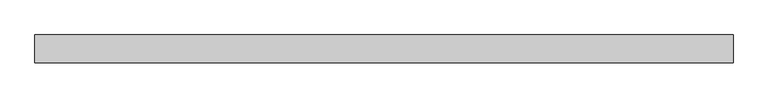
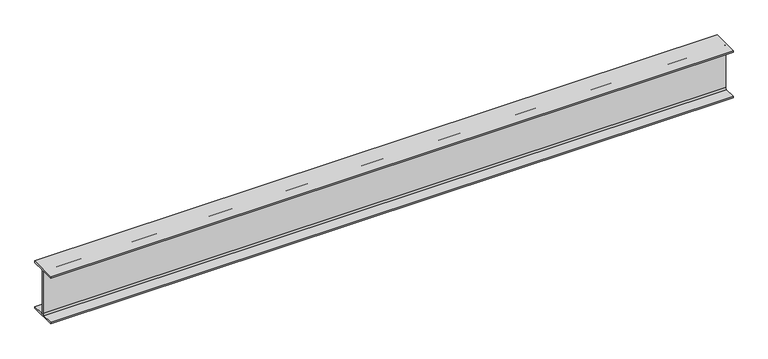
"""IFC4 building model written with IfcOpenShell, lengths in millimetres: beam geometry, Old_Steel Beam_H-KSD3502 : H_SB_ASB_H-250×125x6x9."""

import ifcopenshell
import ifcopenshell.guid

model = None  # the IFC model being written
_history = None  # IfcOwnerHistory: only IFC2X3 demands one
_inside = {}  # id of a spatial element -> (the spatial element, [elements in it])
_under = {}  # id of a project, library or spatial element -> (it, [spatial elements below it])
_declared = {}  # id of a project -> (the project, [libraries it declares])
_typed = {}  # id of a type object -> (the type object, [elements of that type])
_made_of = {}  # id of a material, layer set ... -> (it, [elements and type objects made of it])


def new_model(schema):
    """Start an empty IFC model of exactly this schema.

    Asked for "IFC4X3", IfcOpenShell would pick the latest addendum, in which some entities
    have other attributes; the version numbers below select the first issue.
    IFC2X3 requires an IfcOwnerHistory on every rooted entity: one is made here for all.
    """
    global model, _history
    if schema == "IFC4X3":
        model = ifcopenshell.file(schema_version=(4, 3, 0, 0))
    else:
        model = ifcopenshell.file(schema=schema)
    _inside.clear()
    _under.clear()
    _declared.clear()
    _typed.clear()
    _made_of.clear()
    _history = None
    if model.schema == "IFC2X3":
        org = make("IfcOrganization", Name="unknown")
        user = make(
            "IfcPersonAndOrganization",
            ThePerson=make("IfcPerson", FamilyName="unknown"),
            TheOrganization=org,
        )
        app = make(
            "IfcApplication",
            ApplicationDeveloper=org,
            Version="unknown",
            ApplicationFullName="unknown",
            ApplicationIdentifier="unknown",
        )
        _history = make(
            "IfcOwnerHistory",
            OwningUser=user,
            OwningApplication=app,
            ChangeAction="ADDED",
            CreationDate=0,
        )
    return model


def make(cls, **values):
    """One entity of the class cls with the attributes given. An attribute that is None is left unset."""
    return model.create_entity(
        cls, **{name: value for name, value in values.items() if value is not None}
    )


def rooted(cls, **values):
    """An entity with a GlobalId (a new one), such as an element, a storey or a relation."""
    return make(cls, GlobalId=ifcopenshell.guid.new(), OwnerHistory=_history, **values)


def si_unit(unit_type, name, prefix=None):
    """IfcSIUnit, for example si_unit("LENGTHUNIT", "METRE", prefix="MILLI")."""
    return make("IfcSIUnit", UnitType=unit_type, Prefix=prefix, Name=name)


def assignment(units):
    """IfcUnitAssignment: the units of a project."""
    return None if units is None else make("IfcUnitAssignment", Units=units)


def point(xyz):
    """IfcCartesianPoint."""
    return None if xyz is None else make("IfcCartesianPoint", Coordinates=xyz)


def direction(xyz):
    """IfcDirection."""
    return None if xyz is None else make("IfcDirection", DirectionRatios=xyz)


def frame(location, z_axis=None, x_axis=None):
    """IfcAxis2Placement3D, a coordinate frame: its origin and axes. An axis left out is left unset."""
    return make(
        "IfcAxis2Placement3D",
        Location=point(location),
        Axis=direction(z_axis),
        RefDirection=direction(x_axis),
    )


def frame_2d(location, x_axis=None):
    """IfcAxis2Placement2D, a coordinate frame in the plane: its origin and x axis."""
    return make(
        "IfcAxis2Placement2D", Location=point(location), RefDirection=direction(x_axis)
    )


def origin():
    """The frame at (0, 0, 0) with its axes left unset."""
    return frame((0.0, 0.0, 0.0))


def place(relative_to, where):
    """IfcLocalPlacement: puts the frame where relative to a parent placement (None: the world)."""
    return make(
        "IfcLocalPlacement", PlacementRelTo=relative_to, RelativePlacement=where
    )


def context(
    kind, dimensions, precision=None, world=None, true_north=None, identifier=None
):
    """IfcGeometricRepresentationContext, for example the 3D "Model" context."""
    return make(
        "IfcGeometricRepresentationContext",
        ContextIdentifier=identifier,
        ContextType=kind,
        CoordinateSpaceDimension=dimensions,
        Precision=precision,
        WorldCoordinateSystem=world,
        TrueNorth=true_north,
    )


def project(units=None, contexts=None):
    """IfcProject with its units and contexts."""
    return rooted(
        "IfcProject",
        Name="project",
        RepresentationContexts=contexts,
        UnitsInContext=assignment(units),
    )


def spatial(cls, under=None, at=None, **own):
    """A site, building, storey or space (cls), placed at a placement, below another one or the project."""
    s = rooted(cls, ObjectPlacement=at, **own)
    if under is not None:
        _under.setdefault(under.id(), (under, []))[1].append(s)
    return s


def polyline(points):
    """IfcPolyline through the points."""
    return make("IfcPolyline", Points=[point(p) for p in points])


def circle_curve(where, radius):
    """IfcCircle in the frame where."""
    return make("IfcCircle", Position=where, Radius=radius)


def trimmed(basis, trim1, trim2, sense, master):
    """IfcTrimmedCurve: the piece of a basis curve between two trims."""
    return make(
        "IfcTrimmedCurve",
        BasisCurve=basis,
        Trim1=trim1,
        Trim2=trim2,
        SenseAgreement=sense,
        MasterRepresentation=master,
    )


def segment(curve, same_sense, transition):
    """IfcCompositeCurveSegment."""
    return make(
        "IfcCompositeCurveSegment",
        Transition=transition,
        SameSense=same_sense,
        ParentCurve=curve,
    )


def composite_curve(segments, self_intersect=None):
    """IfcCompositeCurve: segments joined end to end."""
    return make("IfcCompositeCurve", Segments=segments, SelfIntersect=self_intersect)


def outline(outer, holes=None, kind="AREA"):
    """IfcArbitraryClosedProfileDef: a profile drawn as a closed curve; with holes, ...WithVoids."""
    if holes is None:
        return make("IfcArbitraryClosedProfileDef", ProfileType=kind, OuterCurve=outer)
    return make(
        "IfcArbitraryProfileDefWithVoids",
        ProfileType=kind,
        OuterCurve=outer,
        InnerCurves=holes,
    )


def extrude(swept, where, along, depth):
    """IfcExtrudedAreaSolid: the profile swept, set in the frame where, extruded along a direction by depth."""
    return make(
        "IfcExtrudedAreaSolid",
        SweptArea=swept,
        Position=where,
        ExtrudedDirection=direction(along),
        Depth=depth,
    )


def shape(context_of_items, identifier, shape_type, items):
    """IfcShapeRepresentation: the items that make up one representation, for example the "Body"."""
    return make(
        "IfcShapeRepresentation",
        ContextOfItems=context_of_items,
        RepresentationIdentifier=identifier,
        RepresentationType=shape_type,
        Items=items,
    )


def source(mapping_origin, context_of_items, identifier, shape_type, items):
    """IfcRepresentationMap: a shape defined once, which mapped items show again and again."""
    return make(
        "IfcRepresentationMap",
        MappingOrigin=mapping_origin,
        MappedRepresentation=shape(context_of_items, identifier, shape_type, items),
    )


def transform(
    local_origin,
    x_axis=None,
    y_axis=None,
    z_axis=None,
    scale=None,
    scale2=None,
    scale3=None,
    uniform=True,
):
    """IfcCartesianTransformationOperator3D, or its non-uniform kind. x_axis, y_axis, z_axis: its Axis1, 2, 3."""
    if uniform:
        return make(
            "IfcCartesianTransformationOperator3D",
            Axis1=direction(x_axis),
            Axis2=direction(y_axis),
            LocalOrigin=point(local_origin),
            Scale=scale,
            Axis3=direction(z_axis),
        )
    return make(
        "IfcCartesianTransformationOperator3DnonUniform",
        Axis1=direction(x_axis),
        Axis2=direction(y_axis),
        LocalOrigin=point(local_origin),
        Scale=scale,
        Axis3=direction(z_axis),
        Scale2=scale2,
        Scale3=scale3,
    )


def mapped(mapping_source, mapping_target):
    """IfcMappedItem: shows the shape of a source again, moved by a transform."""
    return make(
        "IfcMappedItem", MappingSource=mapping_source, MappingTarget=mapping_target
    )


def made_of(thing, what):
    """Note that an element or type object is made of a material, layer set ...; save() writes the relation."""
    if what is not None:
        _made_of.setdefault(what.id(), (what, []))[1].append(thing)
    return thing


def element(
    cls,
    number,
    at=None,
    inside=None,
    cuts=None,
    type_object=None,
    material=None,
    context=None,
    identifier="Body",
    shape_type=None,
    held_by="IfcProductDefinitionShape",
    body=None,
    shapes=None,
    **own,
):
    """One element of the class cls, such as IfcWall. Its Tag is "e" and its number.

    at: its placement. inside: the storey or other place that contains it. cuts: it is an
    opening in that element (IfcRelVoidsElement). A single representation is given by context,
    identifier, shape_type and body (its items); several are given by shapes. held_by: the class
    of the entity that holds the representations. save() writes the other relations.
    """
    e = rooted(cls, Tag="e%d" % number, ObjectPlacement=at, **own)
    if body is not None:
        shapes = [shape(context, identifier, shape_type, body)]
    if shapes is not None:
        e.Representation = make(held_by, Representations=shapes)
    if inside is not None:
        _inside.setdefault(inside.id(), (inside, []))[1].append(e)
    if cuts is not None:
        rooted(
            "IfcRelVoidsElement", RelatingBuildingElement=cuts, RelatedOpeningElement=e
        )
    if type_object is not None:
        _typed.setdefault(type_object.id(), (type_object, []))[1].append(e)
    return made_of(e, material)


def aggregate(whole, parts):
    """IfcRelAggregates: a whole, such as a stair, and the parts it consists of."""
    return rooted("IfcRelAggregates", RelatingObject=whole, RelatedObjects=parts)


def save(model, path):
    """Write the relations noted so far, then the file.

    IfcRelAggregates (storeys below a building ...), IfcRelContainedInSpatialStructure (elements
    in a storey), IfcRelDefinesByType, IfcRelAssociatesMaterial and IfcRelDeclares: one each for
    every whole, place, type object, material and project.
    """
    for whole, parts in _under.values():
        aggregate(whole, parts)
    for where, things in _inside.values():
        rooted(
            "IfcRelContainedInSpatialStructure",
            RelatedElements=things,
            RelatingStructure=where,
        )
    for kind, things in _typed.values():
        rooted("IfcRelDefinesByType", RelatedObjects=things, RelatingType=kind)
    for what, things in _made_of.values():
        rooted("IfcRelAssociatesMaterial", RelatedObjects=things, RelatingMaterial=what)
    for by, libraries in _declared.values():
        rooted("IfcRelDeclares", RelatingContext=by, RelatedDefinitions=libraries)
    model.write(path)


def beam_10e9c193(model_context):
    return source(origin(), model_context, "Body", "SweptSolid", [
        extrude(outline(composite_curve([segment(polyline([(82.5, -141.5), (82.5, -151.7), (-82.5, -151.7), (-82.5, -141.5), (-11.9, -141.5)]), True, "CONTINUOUS"), segment(trimmed(circle_curve(frame_2d((-11.9, -132.6)), 8.9), [point((-11.9, -141.5))], [point((-3.0, -132.6))], True, "CARTESIAN"), True, "CONTINUOUS"), segment(polyline([(-3.0, -132.6), (-3.0, 132.6)]), True, "CONTINUOUS"), segment(trimmed(circle_curve(frame_2d((-11.9, 132.6)), 8.9), [point((-3.0, 132.6))], [point((-11.9, 141.5))], True, "CARTESIAN"), True, "CONTINUOUS"), segment(polyline([(-11.9, 141.5), (-82.5, 141.5), (-82.5, 151.7), (82.5, 151.7), (82.5, 141.5), (11.9, 141.5)]), True, "CONTINUOUS"), segment(trimmed(circle_curve(frame_2d((11.9, 132.6)), 8.9), [point((11.9, 141.5))], [point((3.0, 132.6))], True, "CARTESIAN"), True, "CONTINUOUS"), segment(polyline([(3.0, 132.6), (3.0, -132.6)]), True, "CONTINUOUS"), segment(trimmed(circle_curve(frame_2d((11.9, -132.6)), 8.9), [point((3.0, -132.6))], [point((11.9, -141.5))], True, "CARTESIAN"), True, "CONTINUOUS"), segment(polyline([(11.9, -141.5), (82.5, -141.5)]), True, "CONTINUOUS")], self_intersect=False)), frame((-2029.8, 0.0, 0.0), z_axis=(1.0, 0.0, 0.0), x_axis=(0.0, 1.0, 0.0)), (0.0, 0.0, 1.0), 4142.0999994),
    ])


if __name__ == "__main__":
    model = new_model("IFC4")
    model_context = context("Model", 3, world=origin())
    ifc_project = project(units=[si_unit("LENGTHUNIT", "METRE", prefix="MILLI")], contexts=[model_context])
    site = spatial("IfcSite", under=ifc_project)
    building = spatial("IfcBuilding", under=site)
    placement = place(None, origin())
    beam_shape = beam_10e9c193(model_context)
    element("IfcBeam", 1, ObjectType="Old_Steel Beam_H-KSD3502 : H_SB_ASB_H-250×125x6x9", at=placement, inside=building, context=model_context, shape_type="MappedRepresentation", body=[
        mapped(beam_shape, transform((0.0, 0.0, 0.0), x_axis=(1.0, 0.0, 0.0), y_axis=(0.0, 1.0, 0.0), z_axis=(0.0, 0.0, 1.0))),
    ])
    save(model, "model.ifc")

# Revit data of these elements
# Type "Old_Steel Beam_H-KSD3502 : H_SB_ASB_H-250×125x6x9"
#   Width = 12.5 cm
#   Web Thickness = 0.6 cm
#   Web Fillet = 1.2 cm
#   Warping Constant = 42539.8 cm⁶
#   Torsional Moment of Inertia = 7.8102 cm⁴
#   Torsional Modulus = 1.0 cm³
#   Section Area = 37.66 cm²
#   Plastic Modulus weak axis = 73.1 cm³
#   Plastic Modulus strong axis = 366.0 cm³
#   Perimeter = 0.97 m²/m
#   Nominal Weight = 29.60 kgf/m
#   Moment of Inertia weak axis = 294.00 cm⁴
#   Moment of Inertia strong axis = 4050.00 cm⁴
#   Height = 25.0 cm
#   Flange Thickness = 0.9 cm
#   Elastic Modulus weak axis = 47.0 cm³
#   Elastic Modulus strong axis = 324.0 cm³
#   Centroid Vertical = 12.5 cm
#   Centroid Horizontal = 6.25 cm
#   Length [instance default] = 1.5240 m
#   Structural Material [instance default] = Steel, 45-345
#   Assembly Code = ""
# Element 1 (IfcBeam, "Old_Steel Beam_H-KSD3502 : H_SB_ASB_H-250×125x6x9")
#   Structural Material = none
# Materials
#   "Steel, 45-345": class "Metal", colour RGB 189 187 185, transparency 0, Description = "Steel 345 MPa", Cost = 0
